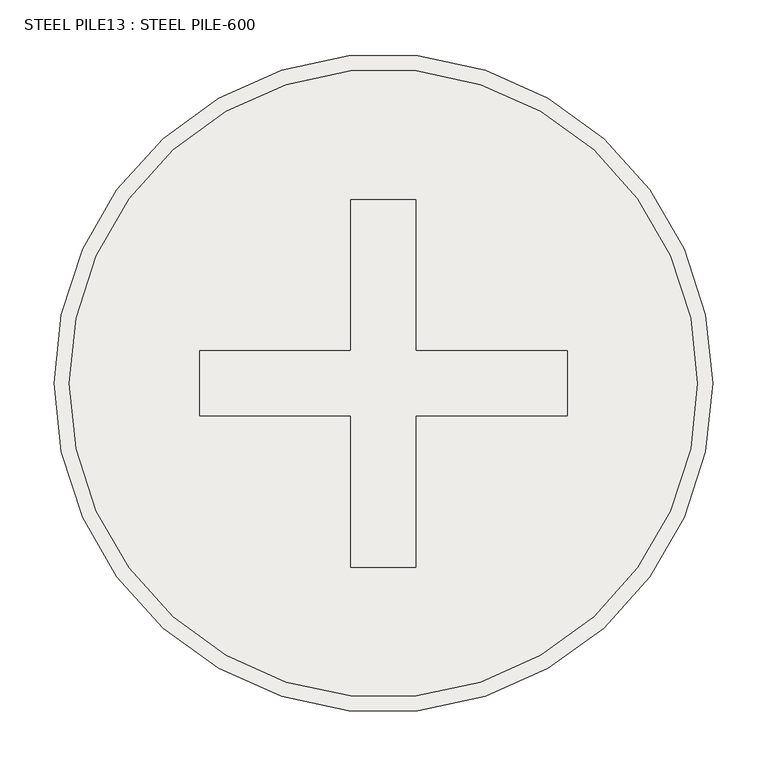
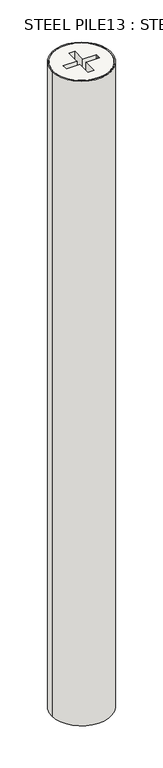
"""IFC4 building model written with IfcOpenShell, lengths in millimetres: slab geometry, STEEL PILE13 : STEEL PILE-600."""

from ifc_helpers import new_model, si_unit, point, frame, frame_2d, origin, place, context, project, spatial, circle_curve, trimmed, segment, composite_curve, outline, extrude, source, transform, mapped, element, save
from ifc_brep_helpers import plane_surface, cylinder_surface, advanced_brep


def steel_pile13_steel_pile_600_05d8cf16(model_context):
    return source(origin(), model_context, "Body", "SolidModel", [
        advanced_brep(
        [(8709.5, 22499.5208589, 150.0), (9290.5, 22499.5208589, 150.0), (8970.0, 22469.5208589, 150.0), (8830.0, 22469.5208589, 150.0), (8830.0, 22499.5208589, 150.0), (8830.0, 22529.5208589, 150.0), (8970.0, 22529.5208589, 150.0), (8970.0, 22669.5208589, 150.0), (9030.0, 22669.5208589, 150.0), (9030.0, 22529.5208589, 150.0), (9170.0, 22529.5208589, 150.0), (9170.0, 22499.5208589, 150.0), (9170.0, 22469.5208589, 150.0), (9030.0, 22469.5208589, 150.0), (9030.0, 22329.5208589, 150.0), (8970.0, 22329.5208589, 150.0), (8709.5, 22499.5208589, -1850.0), (9290.5, 22499.5208589, -1850.0), (8830.0, 22469.5208589, -160.0), (8970.0, 22469.5208589, -160.0), (8970.0, 22329.5208589, -160.0), (9030.0, 22329.5208589, -160.0), (9030.0, 22469.5208589, -160.0), (9170.0, 22469.5208589, -160.0), (9170.0, 22499.5208589, -160.0), (9170.0, 22529.5208589, -160.0), (9030.0, 22529.5208589, -160.0), (9030.0, 22669.5208589, -160.0), (8970.0, 22669.5208589, -160.0), (8970.0, 22529.5208589, -160.0), (8830.0, 22529.5208589, -160.0), (8830.0, 22499.5208589, -160.0)],
        [
            (0, 1, circle_curve(frame((9000.0, 22499.5208589, 150.0), z_axis=(0.0, 0.0, 1.0), x_axis=(1.0, 0.0, 0.0)), 290.5)),
            (1, 0, circle_curve(frame((9000.0, 22499.5208589, 150.0), z_axis=(0.0, 0.0, 1.0), x_axis=(1.0, 0.0, 0.0)), 290.5)),
            (2, 3),
            (3, 4),
            (4, 5),
            (5, 6),
            (6, 7),
            (7, 8),
            (8, 9),
            (9, 10),
            (10, 11),
            (11, 12),
            (12, 13),
            (13, 14),
            (14, 15),
            (15, 2),
            (16, 17, circle_curve(frame((9000.0, 22499.5208589, -1850.0), z_axis=(0.0, 0.0, -1.0), x_axis=(1.0, 0.0, 0.0)), 290.5)),
            (17, 16, circle_curve(frame((9000.0, 22499.5208589, -1850.0), z_axis=(0.0, 0.0, -1.0), x_axis=(1.0, 0.0, 0.0)), 290.5)),
            (0, 16),
            (17, 1),
            (18, 19),
            (19, 20),
            (20, 21),
            (21, 22),
            (22, 23),
            (23, 24),
            (24, 25),
            (25, 26),
            (26, 27),
            (27, 28),
            (28, 29),
            (29, 30),
            (30, 31),
            (31, 18),
            (18, 3),
            (2, 19),
            (15, 20),
            (14, 21),
            (13, 22),
            (12, 23),
            (11, 24),
            (10, 25),
            (9, 26),
            (8, 27),
            (7, 28),
            (6, 29),
            (5, 30),
            (4, 31),
        ],
        [
            plane_surface(frame((9290.5, 22499.5208589, 150.0), z_axis=(0.0, 0.0, 1.0), x_axis=(0.0, 1.0, 0.0))),
            plane_surface(frame((9290.5, 22499.5208589, -1850.0), z_axis=(0.0, 0.0, -1.0), x_axis=(0.0, -1.0, 0.0))),
            cylinder_surface(frame((9000.0, 22499.5208589, -1850.0), z_axis=(0.0, 0.0, 1.0), x_axis=(1.0, 0.0, 0.0)), 290.5),
            plane_surface(frame((8830.0, 22469.5208589, -160.0), z_axis=(0.0, 0.0, 1.0), x_axis=(-1.0, 0.0, 0.0))),
            plane_surface(frame((8830.0, 22469.5208589, 160.0), z_axis=(0.0, 1.0, 0.0), x_axis=(0.0, 0.0, -1.0))),
            plane_surface(frame((8970.0, 22469.5208589, 160.0), z_axis=(1.0, 0.0, 0.0), x_axis=(0.0, 0.0, -1.0))),
            plane_surface(frame((8970.0, 22329.5208589, 160.0), z_axis=(0.0, 1.0, 0.0), x_axis=(0.0, 0.0, -1.0))),
            plane_surface(frame((9030.0, 22329.5208589, 160.0), z_axis=(-1.0, 0.0, 0.0), x_axis=(0.0, 0.0, -1.0))),
            plane_surface(frame((9030.0, 22469.5208589, 160.0), z_axis=(0.0, 1.0, 0.0), x_axis=(0.0, 0.0, -1.0))),
            plane_surface(frame((9170.0, 22469.5208589, 160.0), z_axis=(-1.0, 0.0, 0.0), x_axis=(0.0, 0.0, -1.0))),
            plane_surface(frame((9170.0, 22499.5208589, 160.0), z_axis=(-1.0, 0.0, 0.0), x_axis=(0.0, 0.0, -1.0))),
            plane_surface(frame((9170.0, 22529.5208589, 160.0), z_axis=(0.0, -1.0, 0.0), x_axis=(0.0, 0.0, -1.0))),
            plane_surface(frame((9030.0, 22529.5208589, 160.0), z_axis=(-1.0, 0.0, 0.0), x_axis=(0.0, 0.0, -1.0))),
            plane_surface(frame((9030.0, 22669.5208589, 160.0), z_axis=(0.0, -1.0, 0.0), x_axis=(0.0, 0.0, -1.0))),
            plane_surface(frame((8970.0, 22669.5208589, 160.0), z_axis=(1.0, 0.0, 0.0), x_axis=(0.0, 0.0, -1.0))),
            plane_surface(frame((8970.0, 22529.5208589, 160.0), z_axis=(0.0, -1.0, 0.0), x_axis=(0.0, 0.0, -1.0))),
            plane_surface(frame((8830.0, 22529.5208589, 160.0), z_axis=(1.0, 0.0, 0.0), x_axis=(0.0, 0.0, -1.0))),
            plane_surface(frame((8830.0, 22499.5208589, 160.0), z_axis=(1.0, 0.0, 0.0), x_axis=(0.0, 0.0, -1.0))),
        ],
        [
            (0, [[1, 2], [3, 4, 5, 6, 7, 8, 9, 10, 11, 12, 13, 14, 15, 16]]),
            (1, [[17, 18]]),
            (2, [[-1, 19, -18, 20]]),
            (2, [[-2, -20, -17, -19]]),
            (3, [[21, 22, 23, 24, 25, 26, 27, 28, 29, 30, 31, 32, 33, 34]]),
            (4, [[-21, 35, -3, 36]]),
            (5, [[-22, -36, -16, 37]]),
            (6, [[-23, -37, -15, 38]]),
            (7, [[-24, -38, -14, 39]]),
            (8, [[-25, -39, -13, 40]]),
            (9, [[-26, -40, -12, 41]]),
            (10, [[-27, -41, -11, 42]]),
            (11, [[-28, -42, -10, 43]]),
            (12, [[-29, -43, -9, 44]]),
            (13, [[-30, -44, -8, 45]]),
            (14, [[-31, -45, -7, 46]]),
            (15, [[-32, -46, -6, 47]]),
            (16, [[-33, -47, -5, 48]]),
            (17, [[-34, -48, -4, -35]]),
        ],
    ),
        extrude(outline(composite_curve([segment(trimmed(circle_curve(frame_2d((9000.0, 22499.5208589)), 304.5), [point((8695.5, 22499.5208589))], [point((9304.5, 22499.5208589))], False, "CARTESIAN"), True, "CONTINUOUS"), segment(trimmed(circle_curve(frame_2d((9000.0, 22499.5208589)), 304.5), [point((9304.5, 22499.5208589))], [point((8695.5, 22499.5208589))], False, "CARTESIAN"), True, "CONTINUOUS")], self_intersect=False), holes=[composite_curve([segment(trimmed(circle_curve(frame_2d((9000.0, 22499.5208589)), 290.5), [point((8709.5, 22499.5208589))], [point((9290.5, 22499.5208589))], True, "CARTESIAN"), True, "CONTINUOUS"), segment(trimmed(circle_curve(frame_2d((9000.0, 22499.5208589)), 290.5), [point((9290.5, 22499.5208589))], [point((8709.5, 22499.5208589))], True, "CARTESIAN"), True, "CONTINUOUS")], self_intersect=False)]), frame((0.0, 0.0, -6850.0), z_axis=(0.0, 0.0, 1.0), x_axis=(1.0, 0.0, 0.0)), (0.0, 0.0, 1.0), 7000.0),
    ])


if __name__ == "__main__":
    model = new_model("IFC4")
    model_context = context("Model", 3, world=origin())
    ifc_project = project(units=[si_unit("LENGTHUNIT", "METRE", prefix="MILLI")], contexts=[model_context])
    site = spatial("IfcSite", under=ifc_project)
    building = spatial("IfcBuilding", under=site)
    placement = place(None, origin())
    steel_pile13_steel_pile_600_shape = steel_pile13_steel_pile_600_05d8cf16(model_context)
    element("IfcSlab", 1, ObjectType="STEEL PILE13 : STEEL PILE-600", at=placement, inside=building, context=model_context, shape_type="MappedRepresentation", body=[
        mapped(steel_pile13_steel_pile_600_shape, transform((0.0, 0.0, 0.0), x_axis=(1.0, 0.0, 0.0), y_axis=(0.0, 1.0, 0.0), z_axis=(0.0, 0.0, 1.0))),
    ])
    save(model, "model.ifc")
